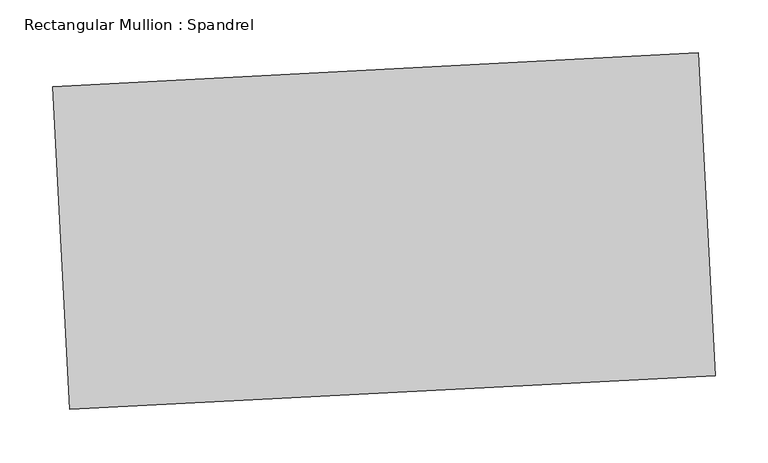
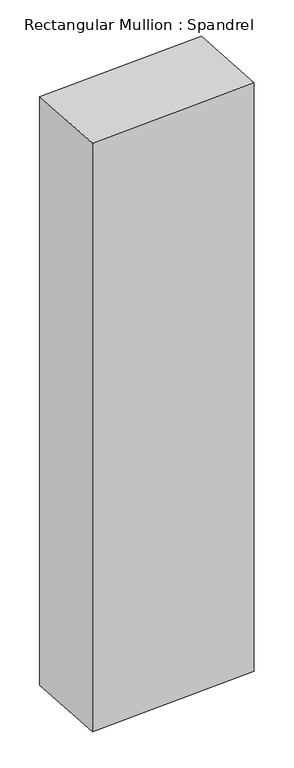
"""IFC4 building model written with IfcOpenShell, lengths in millimetres: member geometry, Rectangular Mullion : Spandrel."""

import ifcopenshell
import ifcopenshell.guid

model = None  # the IFC model being written
_history = None  # IfcOwnerHistory: only IFC2X3 demands one
_inside = {}  # id of a spatial element -> (the spatial element, [elements in it])
_under = {}  # id of a project, library or spatial element -> (it, [spatial elements below it])
_declared = {}  # id of a project -> (the project, [libraries it declares])
_typed = {}  # id of a type object -> (the type object, [elements of that type])
_made_of = {}  # id of a material, layer set ... -> (it, [elements and type objects made of it])


def new_model(schema):
    """Start an empty IFC model of exactly this schema.

    Asked for "IFC4X3", IfcOpenShell would pick the latest addendum, in which some entities
    have other attributes; the version numbers below select the first issue.
    IFC2X3 requires an IfcOwnerHistory on every rooted entity: one is made here for all.
    """
    global model, _history
    if schema == "IFC4X3":
        model = ifcopenshell.file(schema_version=(4, 3, 0, 0))
    else:
        model = ifcopenshell.file(schema=schema)
    _inside.clear()
    _under.clear()
    _declared.clear()
    _typed.clear()
    _made_of.clear()
    _history = None
    if model.schema == "IFC2X3":
        org = make("IfcOrganization", Name="unknown")
        user = make(
            "IfcPersonAndOrganization",
            ThePerson=make("IfcPerson", FamilyName="unknown"),
            TheOrganization=org,
        )
        app = make(
            "IfcApplication",
            ApplicationDeveloper=org,
            Version="unknown",
            ApplicationFullName="unknown",
            ApplicationIdentifier="unknown",
        )
        _history = make(
            "IfcOwnerHistory",
            OwningUser=user,
            OwningApplication=app,
            ChangeAction="ADDED",
            CreationDate=0,
        )
    return model


def make(cls, **values):
    """One entity of the class cls with the attributes given. An attribute that is None is left unset."""
    return model.create_entity(
        cls, **{name: value for name, value in values.items() if value is not None}
    )


def rooted(cls, **values):
    """An entity with a GlobalId (a new one), such as an element, a storey or a relation."""
    return make(cls, GlobalId=ifcopenshell.guid.new(), OwnerHistory=_history, **values)


def si_unit(unit_type, name, prefix=None):
    """IfcSIUnit, for example si_unit("LENGTHUNIT", "METRE", prefix="MILLI")."""
    return make("IfcSIUnit", UnitType=unit_type, Prefix=prefix, Name=name)


def assignment(units):
    """IfcUnitAssignment: the units of a project."""
    return None if units is None else make("IfcUnitAssignment", Units=units)


def point(xyz):
    """IfcCartesianPoint."""
    return None if xyz is None else make("IfcCartesianPoint", Coordinates=xyz)


def direction(xyz):
    """IfcDirection."""
    return None if xyz is None else make("IfcDirection", DirectionRatios=xyz)


def frame(location, z_axis=None, x_axis=None):
    """IfcAxis2Placement3D, a coordinate frame: its origin and axes. An axis left out is left unset."""
    return make(
        "IfcAxis2Placement3D",
        Location=point(location),
        Axis=direction(z_axis),
        RefDirection=direction(x_axis),
    )


def origin():
    """The frame at (0, 0, 0) with its axes left unset."""
    return frame((0.0, 0.0, 0.0))


def place(relative_to, where):
    """IfcLocalPlacement: puts the frame where relative to a parent placement (None: the world)."""
    return make(
        "IfcLocalPlacement", PlacementRelTo=relative_to, RelativePlacement=where
    )


def context(
    kind, dimensions, precision=None, world=None, true_north=None, identifier=None
):
    """IfcGeometricRepresentationContext, for example the 3D "Model" context."""
    return make(
        "IfcGeometricRepresentationContext",
        ContextIdentifier=identifier,
        ContextType=kind,
        CoordinateSpaceDimension=dimensions,
        Precision=precision,
        WorldCoordinateSystem=world,
        TrueNorth=true_north,
    )


def project(units=None, contexts=None):
    """IfcProject with its units and contexts."""
    return rooted(
        "IfcProject",
        Name="project",
        RepresentationContexts=contexts,
        UnitsInContext=assignment(units),
    )


def spatial(cls, under=None, at=None, **own):
    """A site, building, storey or space (cls), placed at a placement, below another one or the project."""
    s = rooted(cls, ObjectPlacement=at, **own)
    if under is not None:
        _under.setdefault(under.id(), (under, []))[1].append(s)
    return s


def polyline(points):
    """IfcPolyline through the points."""
    return make("IfcPolyline", Points=[point(p) for p in points])


def outline(outer, holes=None, kind="AREA"):
    """IfcArbitraryClosedProfileDef: a profile drawn as a closed curve; with holes, ...WithVoids."""
    if holes is None:
        return make("IfcArbitraryClosedProfileDef", ProfileType=kind, OuterCurve=outer)
    return make(
        "IfcArbitraryProfileDefWithVoids",
        ProfileType=kind,
        OuterCurve=outer,
        InnerCurves=holes,
    )


def extrude(swept, where, along, depth):
    """IfcExtrudedAreaSolid: the profile swept, set in the frame where, extruded along a direction by depth."""
    return make(
        "IfcExtrudedAreaSolid",
        SweptArea=swept,
        Position=where,
        ExtrudedDirection=direction(along),
        Depth=depth,
    )


def shape(context_of_items, identifier, shape_type, items):
    """IfcShapeRepresentation: the items that make up one representation, for example the "Body"."""
    return make(
        "IfcShapeRepresentation",
        ContextOfItems=context_of_items,
        RepresentationIdentifier=identifier,
        RepresentationType=shape_type,
        Items=items,
    )


def source(mapping_origin, context_of_items, identifier, shape_type, items):
    """IfcRepresentationMap: a shape defined once, which mapped items show again and again."""
    return make(
        "IfcRepresentationMap",
        MappingOrigin=mapping_origin,
        MappedRepresentation=shape(context_of_items, identifier, shape_type, items),
    )


def transform(
    local_origin,
    x_axis=None,
    y_axis=None,
    z_axis=None,
    scale=None,
    scale2=None,
    scale3=None,
    uniform=True,
):
    """IfcCartesianTransformationOperator3D, or its non-uniform kind. x_axis, y_axis, z_axis: its Axis1, 2, 3."""
    if uniform:
        return make(
            "IfcCartesianTransformationOperator3D",
            Axis1=direction(x_axis),
            Axis2=direction(y_axis),
            LocalOrigin=point(local_origin),
            Scale=scale,
            Axis3=direction(z_axis),
        )
    return make(
        "IfcCartesianTransformationOperator3DnonUniform",
        Axis1=direction(x_axis),
        Axis2=direction(y_axis),
        LocalOrigin=point(local_origin),
        Scale=scale,
        Axis3=direction(z_axis),
        Scale2=scale2,
        Scale3=scale3,
    )


def mapped(mapping_source, mapping_target):
    """IfcMappedItem: shows the shape of a source again, moved by a transform."""
    return make(
        "IfcMappedItem", MappingSource=mapping_source, MappingTarget=mapping_target
    )


def made_of(thing, what):
    """Note that an element or type object is made of a material, layer set ...; save() writes the relation."""
    if what is not None:
        _made_of.setdefault(what.id(), (what, []))[1].append(thing)
    return thing


def element(
    cls,
    number,
    at=None,
    inside=None,
    cuts=None,
    type_object=None,
    material=None,
    context=None,
    identifier="Body",
    shape_type=None,
    held_by="IfcProductDefinitionShape",
    body=None,
    shapes=None,
    **own,
):
    """One element of the class cls, such as IfcWall. Its Tag is "e" and its number.

    at: its placement. inside: the storey or other place that contains it. cuts: it is an
    opening in that element (IfcRelVoidsElement). A single representation is given by context,
    identifier, shape_type and body (its items); several are given by shapes. held_by: the class
    of the entity that holds the representations. save() writes the other relations.
    """
    e = rooted(cls, Tag="e%d" % number, ObjectPlacement=at, **own)
    if body is not None:
        shapes = [shape(context, identifier, shape_type, body)]
    if shapes is not None:
        e.Representation = make(held_by, Representations=shapes)
    if inside is not None:
        _inside.setdefault(inside.id(), (inside, []))[1].append(e)
    if cuts is not None:
        rooted(
            "IfcRelVoidsElement", RelatingBuildingElement=cuts, RelatedOpeningElement=e
        )
    if type_object is not None:
        _typed.setdefault(type_object.id(), (type_object, []))[1].append(e)
    return made_of(e, material)


def aggregate(whole, parts):
    """IfcRelAggregates: a whole, such as a stair, and the parts it consists of."""
    return rooted("IfcRelAggregates", RelatingObject=whole, RelatedObjects=parts)


def save(model, path):
    """Write the relations noted so far, then the file.

    IfcRelAggregates (storeys below a building ...), IfcRelContainedInSpatialStructure (elements
    in a storey), IfcRelDefinesByType, IfcRelAssociatesMaterial and IfcRelDeclares: one each for
    every whole, place, type object, material and project.
    """
    for whole, parts in _under.values():
        aggregate(whole, parts)
    for where, things in _inside.values():
        rooted(
            "IfcRelContainedInSpatialStructure",
            RelatedElements=things,
            RelatingStructure=where,
        )
    for kind, things in _typed.values():
        rooted("IfcRelDefinesByType", RelatedObjects=things, RelatingType=kind)
    for what, things in _made_of.values():
        rooted("IfcRelAssociatesMaterial", RelatedObjects=things, RelatingMaterial=what)
    for by, libraries in _declared.values():
        rooted("IfcRelDeclares", RelatingContext=by, RelatedDefinitions=libraries)
    model.write(path)


def rectangular_mullion_spandrel_372107e3(model_context):
    return source(origin(), model_context, "Body", "SweptSolid", [
        extrude(outline(polyline([(-617.1582819, 136.2391416), (-8.3937175, 168.1431406), (7.5582819, -136.2391416), (-601.2062825, -168.1431406), (-617.1582819, 136.2391416)])), frame((0.0, 0.0, -2268.2609739), z_axis=(0.0, 0.0, 1.0), x_axis=(1.0, 0.0, 0.0)), (0.0, 0.0, 1.0), 2268.2609739),
    ])


if __name__ == "__main__":
    model = new_model("IFC4")
    model_context = context("Model", 3, world=origin())
    ifc_project = project(units=[si_unit("LENGTHUNIT", "METRE", prefix="MILLI")], contexts=[model_context])
    site = spatial("IfcSite", under=ifc_project)
    building = spatial("IfcBuilding", under=site)
    placement = place(None, origin())
    rectangular_mullion_spandrel_shape = rectangular_mullion_spandrel_372107e3(model_context)
    element("IfcMember", 1, ObjectType="Rectangular Mullion : Spandrel", at=placement, inside=building, context=model_context, shape_type="MappedRepresentation", body=[
        mapped(rectangular_mullion_spandrel_shape, transform((0.0, 0.0, 0.0), x_axis=(1.0, 0.0, 0.0), y_axis=(0.0, 1.0, 0.0), z_axis=(0.0, 0.0, 1.0))),
    ])
    save(model, "model.ifc")

# Revit data of these elements
# Type "Rectangular Mullion : Spandrel"
#   built-in parameter 1007304 = 1 (stored number, unit not read)
#   built-in parameter 1007301 = 1 (stored number, unit not read)
#   built-in parameter 1007300 = 1 (stored number, unit not read)
# Element 1 (IfcMember, "Rectangular Mullion : Spandrel")
#   Materials on its faces: "Aluminum"
# Materials
#   "Aluminum": class "Metal", colour RGB 247 247 247, transparency 0, Description = "Aluminum 6061", Cost = 0
